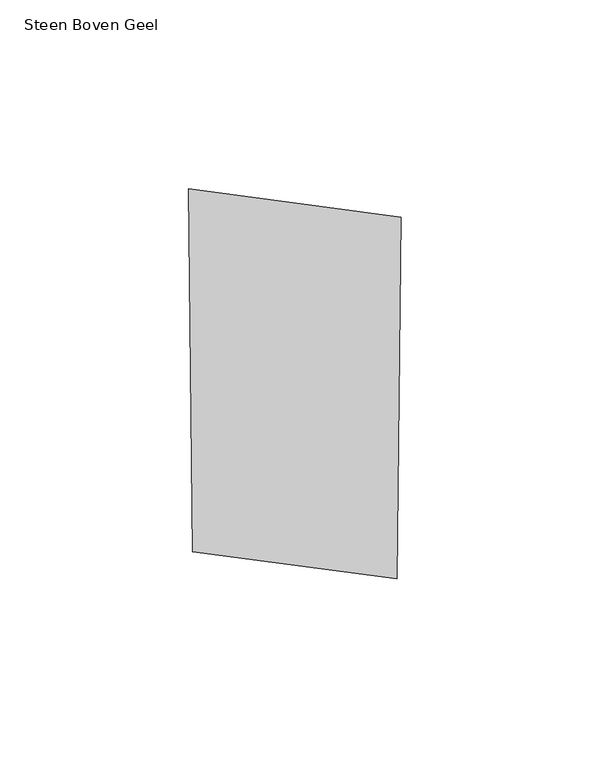
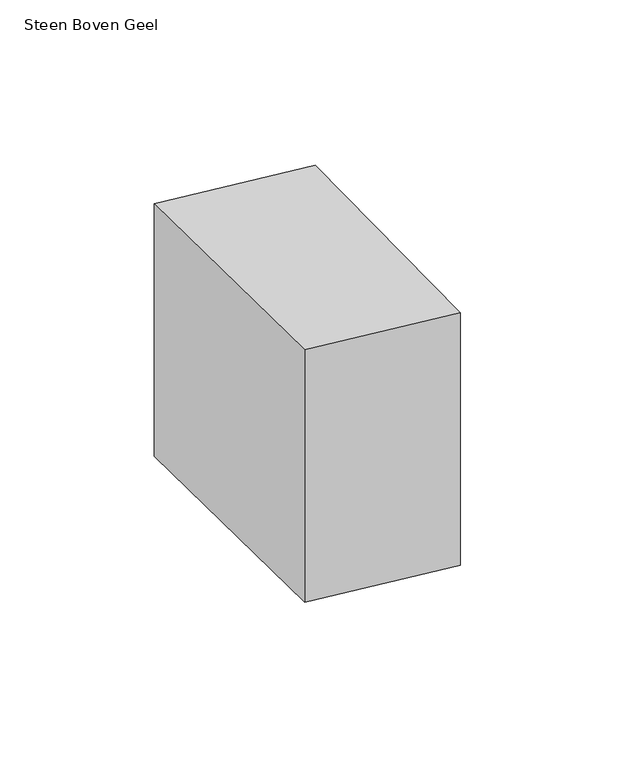
"""IFC4 building model written with IfcOpenShell, lengths in millimetres: proxy geometry, 00_GMA_steen_versie_4 : Steen Boven Geel."""

from ifc_helpers import new_model, si_unit, origin, origin_with_axes, place, context, project, spatial, polyline, outline, extrude, source, transform, mapped, element, save


def steen_boven_geel_a9964f13(model_context):
    return source(origin(), model_context, "Body", "SweptSolid", [
        extrude(outline(polyline([(101.1368384, 119.6252427), (100.1103155, 23.8854918), (46.0330672, 31.0718074), (44.9656685, 127.102594), (101.1368384, 119.6252427)])), origin_with_axes(), (0.0, 0.0, 1.0), 100.0),
    ])


if __name__ == "__main__":
    model = new_model("IFC4")
    model_context = context("Model", 3, world=origin())
    ifc_project = project(units=[si_unit("LENGTHUNIT", "METRE", prefix="MILLI")], contexts=[model_context])
    site = spatial("IfcSite", under=ifc_project)
    building = spatial("IfcBuilding", under=site)
    placement = place(None, origin())
    steen_boven_geel_shape = steen_boven_geel_a9964f13(model_context)
    element("IfcBuildingElementProxy", 1, Name="00_GMA_steen_versie_4 : Steen Boven Geel", ObjectType="00_GMA_steen_versie_4 : Steen Boven Geel", at=placement, inside=building, context=model_context, shape_type="MappedRepresentation", body=[
        mapped(steen_boven_geel_shape, transform((0.0, 0.0, 0.0), x_axis=(1.0, 0.0, 0.0), y_axis=(0.0, 1.0, 0.0), z_axis=(0.0, 0.0, 1.0))),
    ])
    save(model, "model.ifc")

# Revit data of these elements
# Type "00_GMA_steen_versie_4 : Steen Boven Geel"
#   StootVoegHalfBoven [instance default] = 5 mm
#   StootVoegHalf [instance default] = 5 mm
#   StootVoegBreedteOnder = 10 mm
#   StootVoegBreedteBoven = 10 mm
#   Steendikte = 100 mm
#   LintVoegOnderHalf = 5 mm
#   LintVoegOnder = 10 mm
#   LintVoegBovenHalf = 0 mm
#   LintVoegBoven = 0 mm
#   materiaal = 21_steen_geel
#   MateriaalVoeg = none
#   Default Elevation = 0
# Element 1 (IfcBuildingElementProxy, "00_GMA_steen_versie_4 : Steen Boven Geel")
#   Materials on its faces: "21_steen_geel"
# Materials
#   "21_steen_geel": class "Unassigned", colour RGB 202 202 0, transparency 0, Cost = 0
